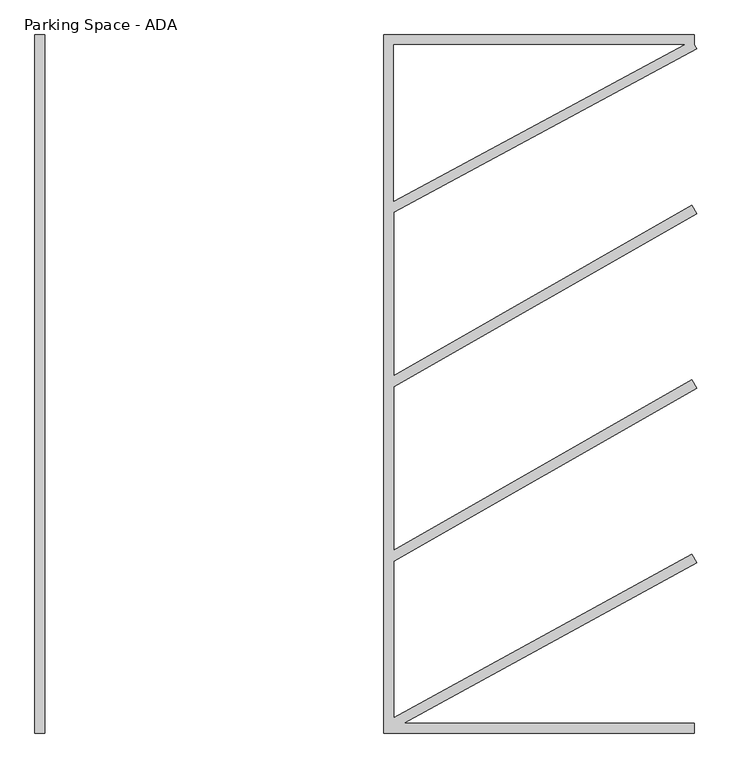
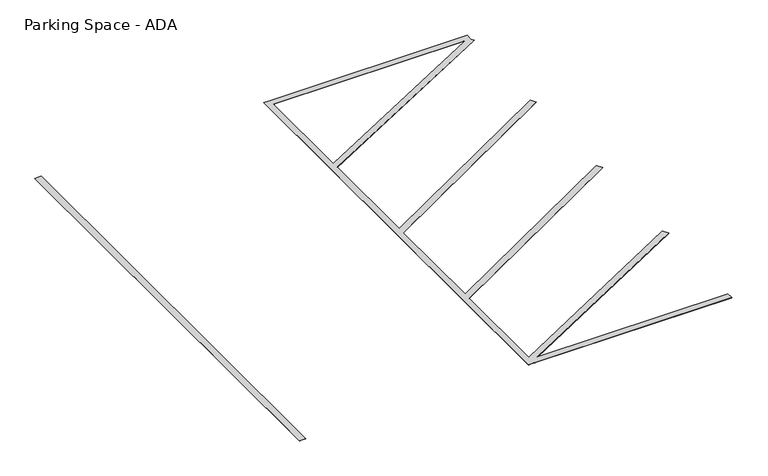
"""IFC4 building model written with IfcOpenShell, lengths in millimetres: proxy geometry, Parking Space - ADA : 9' x 18' (8' Aisle)."""

from ifc_helpers import new_model, si_unit, origin, origin_with_axes, place, context, project, spatial, polyline, outline, extrude, source, transform, mapped, element, save


def parking_space_ada_44d2459f(model_context):
    return source(origin(), model_context, "Body", "SweptSolid", [
        extrude(outline(polyline([(4046.2620479, 859.2253385), (6408.4620479, 859.2253385), (6408.4620479, 783.0253385), (6426.55698, 749.4964937), (4046.2620479, -535.1071205), (4046.2620479, -1818.3215158), (6389.5591543, -479.2945978), (6427.3649414, -545.4547253), (4046.2620479, -1906.0849501), (4046.2620479, -3189.9215158), (6389.5591543, -1850.8945978), (6427.3649414, -1917.0547253), (4046.2620479, -3277.6849501), (4046.2620479, -4507.5218093), (6390.1423254, -3222.1681088), (6426.7817704, -3288.9812143), (4125.4996019, -4550.9746615), (6408.4620479, -4550.9746615), (6408.4620479, -4627.1746615), (4046.2620479, -4627.1746615), (3970.0620479, -4627.1746615), (3970.0620479, 859.2253385), (4046.2620479, 859.2253385)]), holes=[polyline([(6328.2401387, 783.0253385), (4046.2620479, 783.0253385), (4046.2620479, -448.5183931), (6328.2401387, 783.0253385)])]), origin_with_axes(), (0.0, 0.0, 1.0), 1.5875),
        extrude(outline(polyline([(1303.0620479, 859.2253385), (1303.0620479, -4627.1746615), (1226.8620479, -4627.1746615), (1226.8620479, 859.2253385), (1303.0620479, 859.2253385)])), origin_with_axes(), (0.0, 0.0, 1.0), 1.5875),
    ])


if __name__ == "__main__":
    model = new_model("IFC4")
    model_context = context("Model", 3, world=origin())
    ifc_project = project(units=[si_unit("LENGTHUNIT", "METRE", prefix="MILLI")], contexts=[model_context])
    site = spatial("IfcSite", under=ifc_project)
    building = spatial("IfcBuilding", under=site)
    placement = place(None, origin())
    parking_space_ada_shape = parking_space_ada_44d2459f(model_context)
    element("IfcBuildingElementProxy", 1, Name="Parking Space - ADA : 9' x 18' (8' Aisle)", ObjectType="Parking Space - ADA : 9' x 18' (8' Aisle)", at=placement, inside=building, context=model_context, shape_type="MappedRepresentation", body=[
        mapped(parking_space_ada_shape, transform((0.0, 0.0, 0.0), x_axis=(1.0, 0.0, 0.0), y_axis=(0.0, 1.0, 0.0), z_axis=(0.0, 0.0, 1.0))),
    ])
    save(model, "model.ifc")

# Revit data of these elements
# Type "Parking Space - ADA : 9' x 18' (8' Aisle)"
#   Accesible Aisle = 2438.4 mm
#   Length = 5486.4 mm
#   Width = 2743.2 mm
# Element 1 (IfcBuildingElementProxy, "Parking Space - ADA : 9' x 18' (8' Aisle)")
#   Materials on its faces: "Parking Stripe"
# Materials
#   "Parking Stripe": class "Paint", colour RGB 250 250 91, transparency 0, Cost = 0
